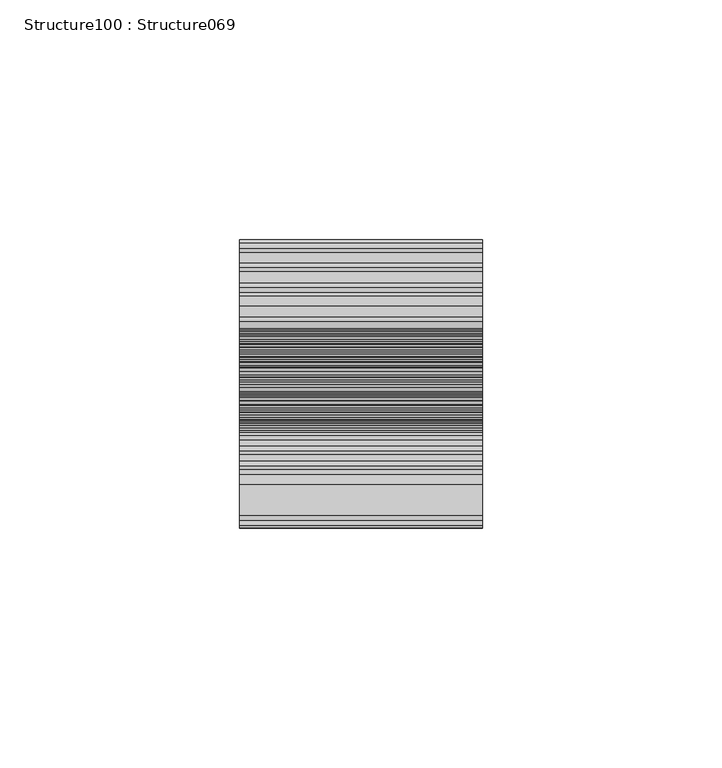
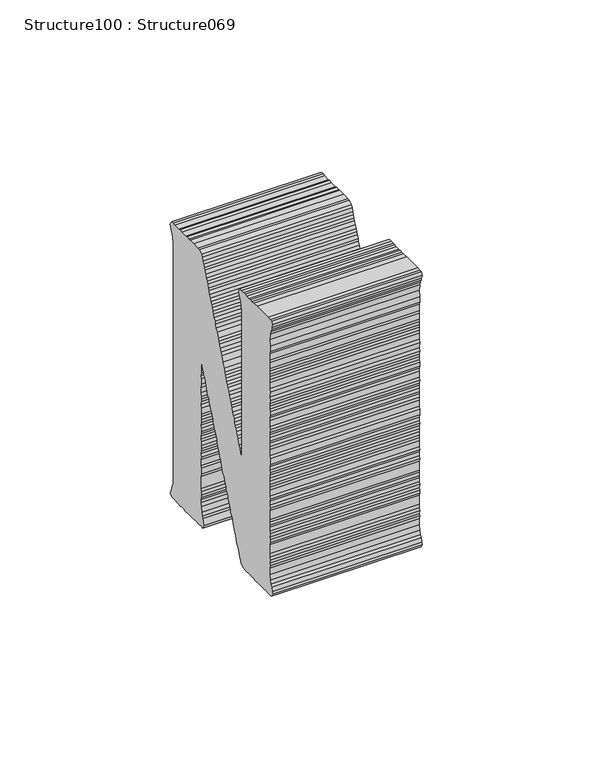
"""IFC4 building model written with IfcOpenShell, lengths in millimetres: proxy geometry, Structure100 : Structure069."""

from ifc_helpers import new_model, si_unit, frame, origin, place, context, project, spatial, polyline, outline, extrude, source, transform, mapped, element, save


def structure100_structure069_ddb158e7(model_context):
    return source(origin(), model_context, "Body", "SweptSolid", [
        extrude(outline(polyline([(1.8366799, 0.0), (3.1712942, 0.2003909), (3.9678799, 0.2224656), (6.1339986, 0.7044793), (7.2010362, -0.1051671), (6.9235449, -1.1141612), (6.9103347, -2.1601811), (6.6008944, -4.347663), (6.6194392, -5.1387182), (6.4553745, -6.298517), (6.2008497, -7.1756413), (6.164673, -8.353531), (5.8912652, -10.286294), (5.5038773, -11.150014), (5.322519, -12.4320636), (5.4724816, -13.2467403), (5.3278037, -14.2694911), (4.776401, -16.2926574), (4.4850018, -18.3526038), (3.4817959, -18.9944509), (2.4116511, -18.1940677), (1.5481838, -17.8074343), (0.6787273, -17.4199537), (-0.4031239, -16.7429712), (-2.5708599, -16.3015648), (-3.6179366, -16.2882051), (-4.4817063, -15.9011696), (-5.5316583, -15.8827315), (-7.7145603, -15.573939), (-8.6005421, -15.3185207), (-9.646971, -15.300581), (-13.7622836, -14.7184305), (-14.8072465, -14.7053698), (-15.8412712, -14.5590971), (-16.8492085, -14.2817554), (-18.0093595, -14.1176409), (-19.0175923, -13.844929), (-20.0827102, -13.9591049), (-20.8238767, -13.5894127), (-22.015121, -13.6857468), (-23.1509461, -13.3903141), (-24.0757719, -13.394248), (-27.2905847, -12.9394818), (-28.3002834, -12.6618909), (-29.3265574, -12.5167146), (-30.11962, -12.5392877), (-31.3691672, -12.0976802), (-33.4665482, -12.0658325), (-34.4928222, -11.9206562), (-35.3742808, -11.6612061), (-36.5167429, -11.3695062), (-37.5628196, -11.3516163), (-38.4452783, -11.0966964), (-39.363467, -11.0968974), (-40.5405456, -11.0651477), (-42.5969688, -10.7742469), (-43.5925018, -10.3685722), (-44.619128, -10.2233461), (-45.6838937, -10.3375718), (-46.5473111, -9.9505861), (-47.870671, -10.0282311), (-48.6260031, -9.7866228), (-49.6713184, -9.7735123), (-50.7947393, -9.3497466), (-51.9916205, -9.4452833), (-52.7232746, -9.0769368), (-53.9145189, -9.1732708), (-54.7818118, -8.7857369), (-56.1069332, -8.8631328), (-58.1672318, -8.5716838), (-59.0250123, -8.1854955), (-60.0943579, -8.2990733), (-61.0856633, -7.8939966), (-61.9896861, -7.7661139), (-63.3091707, -7.8443072), (-64.300476, -7.4392305), (-65.1151027, -7.5888408), (-66.1230399, -7.311499), (-67.2591607, -7.0206962), (-68.4193117, -6.8565817), (-69.3565418, -6.9888485), (-70.5114082, -6.8254816), (-71.2486992, -6.4563377), (-72.4268915, -6.4197588), (-73.4774913, -6.4059006), (-74.6320055, -6.2425835), (-75.382053, -6.0017228), (-76.673615, -5.8190189), (-77.7189303, -5.8059084), (-78.7109403, -5.4007321), (-79.7608922, -5.382294), (-80.6391233, -5.1279721), (-81.7077643, -5.2416496), (-82.829776, -4.8180832), (-83.6348904, -4.9690391), (-84.9045926, -4.6546682), (-85.695189, -4.6775901), (-88.0278455, -4.4773416), (-88.9646734, -4.609306), (-90.2108917, -5.0917202), (-91.0201978, -5.2316616), (-92.1011932, -5.4733198), (-93.1586381, -4.5399738), (-93.1206999, -3.3623333), (-92.7520508, -2.6310813), (-92.4419626, -0.4390194), (-92.5752795, 0.4933283), (-92.1872438, 1.3616281), (-91.8605099, 3.6713609), (-91.9924812, 4.6132209), (-91.587102, 5.604124), (-91.7377125, 6.4142206), (-91.4463133, 8.4741669), (-90.858928, 10.7516998), (-90.7315437, 11.6521997), (-89.7588844, 12.9570716), (-88.9368785, 13.2299759), (-87.6082839, 13.3065211), (-86.6587493, 13.5664164), (-85.7042326, 13.8259662), (-84.8931789, 13.9757224), (-83.7762507, 14.4713949), (-82.5614281, 14.6937625), (-81.6062067, 14.9532126), (-80.6633896, 15.0843297), (-79.4369103, 15.4297457), (-78.6501893, 15.4532158), (-77.5449108, 15.8208079), (-76.462154, 16.0622168), (-75.3815538, 16.2985406), (-74.534172, 16.7076455), (-73.5973441, 16.8396099), (-72.5103596, 17.0804208), (-71.687656, 17.3582575), (-70.4908177, 17.4484098), (-69.5003682, 17.9619739), (-68.5634905, 18.0942906), (-67.3684206, 18.1897241), (-66.2493787, 18.6850975), (-64.4672261, 19.2217862), (-63.510293, 19.4806349), (-62.4663801, 19.4626916), (-61.3649772, 19.8308319), (-60.1522683, 20.0534986), (-59.1790557, 20.4401319), (-57.1602185, 20.8082206), (-55.3756066, 21.3495925), (-54.1625454, 21.5722094), (-53.227113, 21.6943091), (-52.2712438, 21.9583392), (-51.0789855, 22.0491395), (-50.3414505, 22.603871), (-49.2971852, 22.585878), (-48.3063834, 23.0993922), (-47.1095521, 23.1945765), (-46.0035261, 23.5674532), (-45.0532801, 23.8222167), (-44.0981086, 24.0813146), (-43.3078576, 24.0992543), (-41.9481697, 24.436248), (-40.9757116, 24.8226288), (-40.0212378, 25.0767942), (-38.9505328, 25.1898204), (-37.8872262, 25.3038932), (-37.0641205, 25.5820323), (-35.977538, 25.8225407), (-34.8771851, 26.1857986), (-34.031515, 26.595505), (-32.0246798, 26.8355632), (-31.0761952, 27.0905759), (-29.7162049, 27.4271676), (-28.755699, 27.6858701), (-29.9756481, 28.3773569), (-32.0655947, 28.4185743), (-34.1262456, 28.7100732), (-34.8632205, 29.0687509), (-36.0194961, 29.2323172), (-37.0630636, 29.2552425), (-38.22709, 29.4199052), (-39.2734691, 29.4381973), (-40.0065686, 29.7963269), (-41.0741166, 29.6929162), (-42.0672194, 30.0878257), (-43.0994827, 30.2338493), (-44.2889293, 30.1476823), (-45.171438, 30.4022499), (-46.4404218, 30.7064572), (-47.2320888, 30.6937487), (-48.2724787, 30.7111936), (-49.4015725, 31.1253403), (-50.4469016, 31.1485148), (-51.4562342, 31.415992), (-53.5165329, 31.707441), (-54.5837286, 31.6039805), (-56.59923, 32.1435181), (-57.3771267, 32.253559), (-58.4411516, 32.14965), (-59.7094377, 32.4587895), (-60.4996887, 32.4408498), (-61.5224395, 32.5855277), (-62.7787167, 33.0176658), (-63.5827382, 32.8769768), (-65.6433891, 33.1684756), (-66.9116752, 33.4776151), (-68.9719739, 33.7690641), (-69.8495432, 34.017902), (-70.9188528, 33.9147406), (-71.8010091, 34.1692583), (-72.9555232, 34.3325754), (-74.1022561, 34.6194891), (-75.1479374, 34.6427134), (-75.9029036, 34.874208), (-78.2468644, 34.9513581), (-79.2459565, 35.3471149), (-80.2718781, 35.4922413), (-82.2586151, 35.3840994), (-83.4695623, 35.1611835), (-84.4106677, 35.0294649), (-85.6374925, 34.6790667), (-86.7195018, 34.4429424), (-87.7897033, 35.2480052), (-87.5340788, 36.1303644), (-87.3520228, 37.4173463), (-87.3349372, 38.462818), (-86.9711775, 39.2001521), (-86.7891714, 40.4867817), (-86.8981624, 41.5504475), (-86.5344027, 42.2877815), (-86.3890769, 43.3151124), (-86.3520443, 45.4110413), (-85.4425121, 51.8406668), (-85.0420721, 52.8372997), (-85.0228229, 53.8828246), (-83.9355358, 54.1232334), (-82.7042823, 53.5548448), (-81.9482524, 53.3181688), (-80.8667964, 52.6358518), (-79.8927349, 52.1088765), (-77.7419401, 51.5451693), (-75.6456589, 51.5080868), (-73.7185328, 51.2354764), (-72.7226045, 50.8351361), (-70.5397026, 50.5263436), (-69.7476901, 50.5440342), (-67.5556282, 50.233946), (-66.5508686, 49.9620848), (-65.5062511, 49.944042), (-64.6184579, 49.6887268), (-63.5738403, 49.6706839), (-62.4316806, 49.3793861), (-60.3770189, 49.0887345), (-59.3066593, 49.1967786), (-57.2879802, 48.6517603), (-56.2200868, 48.7601532), (-55.0832117, 48.469603), (-54.1777794, 48.3415209), (-53.0409043, 48.0509707), (-52.2365374, 48.196642), (-50.9442707, 48.0138384), (-50.0804581, 47.6321872), (-49.0358406, 47.6141443), (-46.8473017, 47.3045545), (-45.9252875, 47.3038551), (-44.7887646, 47.0133547), (-44.0383716, 46.7774761), (-43.0064608, 46.6315024), (-41.8318415, 46.5950695), (-40.9493329, 46.3405019), (-39.7733044, 46.3038697), (-38.6307924, 46.0125221), (-36.576483, 45.7219203), (-35.6400005, 45.8489025), (-33.5797018, 45.5574535), (-32.7095476, 45.1749052), (-31.4109159, 45.1209296), (-30.6245403, 45.1394176), (-29.6282597, 44.7390274), (-28.5822329, 44.7207852), (-27.5538452, 44.5753099), (-26.2816836, 44.2656221), (-25.4953081, 44.2841101), (-24.2249081, 43.9746715), (-22.1663711, 43.6834717), (-21.2298885, 43.8104539), (-20.3657236, 43.4287528), (-19.059341, 43.3736808), (-18.0094388, 43.3548904), (-17.1329195, 43.10117), (-13.9177544, 42.646354), (-13.0299613, 42.3910388), (-11.8574559, 42.354905), (-11.1010736, 42.1181791), (-9.7968049, 42.0634062), (-9.0104293, 42.0818941), (-7.7421432, 41.7727545), (-6.8180151, 41.7717561), (-5.7917412, 41.6265798), (-4.9275762, 41.2448787), (-1.7124111, 40.7900627), (-0.5342688, 40.7531315), (0.3782332, 40.7537777), (1.5263822, 40.4616327), (2.3127577, 40.4801206), (3.4348124, 40.0619386), (5.6233512, 39.7523488), (7.4599813, 39.7519965), (8.7945956, 39.9523874), (9.6459027, 40.3612965), (10.9833286, 40.5663208), (11.7940302, 40.7161269), (12.8430266, 39.778945), (12.7156921, 38.8787974), (12.715498, 37.9552743), (12.4063016, 36.6916678), (12.2789173, 35.7911679), (11.982737, 34.6500582), (12.1340951, 33.8452463), (11.8234534, 32.5714229), (11.6606399, 30.4983179), (11.2725543, 29.6296657), (11.3872321, 28.5655549), (10.9638616, 27.4474684), (10.8544685, 26.6741518), (10.9691462, 25.610041), (10.6771936, 24.4683331), (10.5498591, 23.5681856), (9.4634279, 22.4091362), (8.5124841, 22.1494403), (7.3948084, 21.6484833), (6.4706803, 21.6494817), (5.2621923, 21.431249), (4.2826949, 21.040833), (3.3154715, 20.6533524), (2.1186401, 20.558168), (1.0144118, 20.1954585), (-0.8952764, 19.6768108), (-1.8472703, 19.4122326), (-2.6424604, 19.4000225), (-3.9777726, 19.1946993), (-4.8065152, 18.9173575), (-5.9244934, 18.4168027), (-6.8426322, 18.4169539), (-7.9493198, 18.0495612), (-8.9041889, 17.7900613), (-9.8713623, 17.402933), (-11.0540779, 17.4354801), (-11.8944274, 17.0354423), (-13.000101, 16.6625158), (-13.9147167, 16.6621687), (-15.0161129, 16.2889964), (-15.8236573, 16.1488057), (-16.9067168, 15.9077989), (-17.9021415, 15.3895482), (-19.94002, 14.8893938), (-20.9846376, 14.9074366), (-22.085738, 14.5388943), (-22.9183063, 14.262453), (-24.2373886, 14.1845622), (-26.0371803, 13.5206404), (-27.1258766, 13.2804309), (-28.0443677, 13.2806321), (-29.2528557, 13.0623993), (-30.079787, 12.7851608), (-31.1812329, 12.4116362), (-31.990173, 12.2615808), (-33.2413305, 11.7848965), (-34.2873573, 11.8031387), (-35.3923332, 11.4351444), (-36.3235242, 11.3023827), (-37.4291479, 10.9298085), (-39.4663786, 10.4342341), (-40.4032064, 10.3022697), (-41.2615472, 9.7750487), (-42.2223557, 9.5167482), (-43.3040488, 9.2701577), (-44.3722945, 9.1618148), (-45.1773591, 9.0112112), (-46.3854949, 8.7929286), (-47.5112736, 8.2931179), (-48.4484538, 8.1612034), (-49.2753851, 7.8839647), (-50.3573944, 7.6478404), (-51.4623703, 7.2798462), (-50.4487962, 7.001707), (-49.5334827, 7.0069865), (-48.2419206, 6.8242826), (-47.3601098, 6.5647827), (-46.3514748, 6.2923733), (-45.4333359, 6.2922221), (-43.3726851, 6.0007232), (-42.1043989, 5.6915836), (-40.3037515, 5.4368648), (-38.9977212, 5.3818426), (-38.2106479, 5.4052629), (-37.1970738, 5.1271237), (-36.060551, 4.8366233), (-34.9954828, 4.9504469), (-32.8090579, 4.6411561), (-31.7954837, 4.363017), (-30.8766472, 4.3677981), (-29.740822, 4.0723654), (-28.8526765, 3.8170003), (-27.7897223, 3.9311229), (-26.6330943, 3.7675068), (-25.7477604, 3.5075085), (-24.8694795, 3.2535389), (-23.8372163, 3.1075153), (-22.9190774, 3.1073641), (-21.6324477, 2.925358), (-20.5857232, 2.9120481), (-19.577786, 2.6347064), (-18.6899928, 2.3793912), (-17.6249247, 2.4932147), (-16.5070909, 2.0705988), (-14.4485539, 1.7793989), (-13.5300626, 1.7791979), (-11.469764, 1.4877489), (-10.5876078, 1.2332311), (-6.2122917, 0.6143006), (-5.2997897, 0.6149468), (-4.1149604, 0.5821006), (-3.2204497, 0.4555635), (-2.3513456, 0.0681327), (-1.3247193, -0.0770934), (0.0, 0.0), (1.8366799, 0.0)])), frame((-56111.6093717, 291076.9340177, -368.3266136), z_axis=(-0.9999998917542984, 0.00046528635450596156, 0.0), x_axis=(-6.517039355318693e-05, -0.14006511446573924, -0.9901422925330072)), (0.0, 0.0, 1.0), 50.8),
    ])


if __name__ == "__main__":
    model = new_model("IFC4")
    model_context = context("Model", 3, world=origin())
    ifc_project = project(units=[si_unit("LENGTHUNIT", "METRE", prefix="MILLI")], contexts=[model_context])
    site = spatial("IfcSite", under=ifc_project)
    building = spatial("IfcBuilding", under=site)
    placement = place(None, origin())
    structure100_structure069_shape = structure100_structure069_ddb158e7(model_context)
    element("IfcBuildingElementProxy", 1, Name="Structure100 : Structure069", ObjectType="Structure100 : Structure069", at=placement, inside=building, context=model_context, shape_type="MappedRepresentation", body=[
        mapped(structure100_structure069_shape, transform((0.0, 0.0, 0.0), x_axis=(1.0, 0.0, 0.0), y_axis=(0.0, 1.0, 0.0), z_axis=(0.0, 0.0, 1.0))),
    ])
    save(model, "model.ifc")

# Revit data of these elements
# Type "Structure100 : Structure069"
#   NameOverride = "Structure069"
# Element 1 (IfcBuildingElementProxy, "Structure100 : Structure069")
#   Materials on its faces: "BRUSHED ALUMINUM LETTERING"
# Materials
#   "BRUSHED ALUMINUM LETTERING": class "Unassigned", colour RGB 169 181 186, transparency 0, Cost = 0
